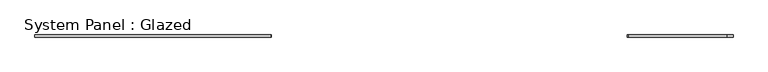
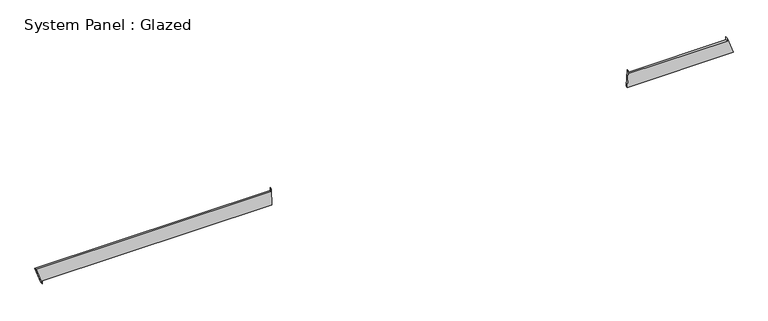
"""IFC4 building model written with IfcOpenShell, lengths in millimetres: plate geometry, System Panel : Glazed."""

from ifc_helpers import new_model, si_unit, frame, origin, place, context, project, spatial, polyline, outline, extrude, source, transform, mapped, element, save


def system_panel_glazed_fa53dddc(model_context):
    return source(origin(), model_context, "Body", "SweptSolid", [
        extrude(outline(polyline([(0.0, -3958.8254362), (35.3553391, -3958.8254362), (35.3553391, -1302.7884729), (234.738189, -1308.1565543), (199.3828499, -1308.1560034), (199.3404739, -4027.6368042), (0.0, -3958.8254362)])), frame((0.0, -49.5, 0.0), z_axis=(0.0, 1.0, 0.0), x_axis=(0.0, 0.0, 1.0)), (0.0, 0.0, 1.0), 25.0),
        extrude(outline(polyline([(35.3553391, 2804.942479), (35.3553391, 4027.6368042), (234.820266, 3959.126507), (199.4649269, 3959.1270579), (199.4471238, 2816.613626), (234.8024629, 2816.6130751), (35.3553391, 2804.942479)])), frame((0.0, -49.5, 0.0), z_axis=(0.0, 1.0, 0.0), x_axis=(0.0, 0.0, 1.0)), (0.0, 0.0, 1.0), 25.0),
    ])


if __name__ == "__main__":
    model = new_model("IFC4")
    model_context = context("Model", 3, world=origin())
    ifc_project = project(units=[si_unit("LENGTHUNIT", "METRE", prefix="MILLI")], contexts=[model_context])
    site = spatial("IfcSite", under=ifc_project)
    building = spatial("IfcBuilding", under=site)
    placement = place(None, origin())
    system_panel_glazed_shape = system_panel_glazed_fa53dddc(model_context)
    element("IfcPlate", 1, ObjectType="System Panel : Glazed", at=placement, inside=building, context=model_context, shape_type="MappedRepresentation", body=[
        mapped(system_panel_glazed_shape, transform((0.0, 0.0, 0.0), x_axis=(1.0, 0.0, 0.0), y_axis=(0.0, 1.0, 0.0), z_axis=(0.0, 0.0, 1.0))),
    ])
    save(model, "model.ifc")

# Revit data of these elements
# Element 1 (IfcPlate, "System Panel : Glazed")
#   Materials on its faces: "Glass"
# Materials
#   "Glass": class "Glass", colour RGB 218 227 224, transparency 0.85, Description = "Soda Lime Glass", Cost = 0
